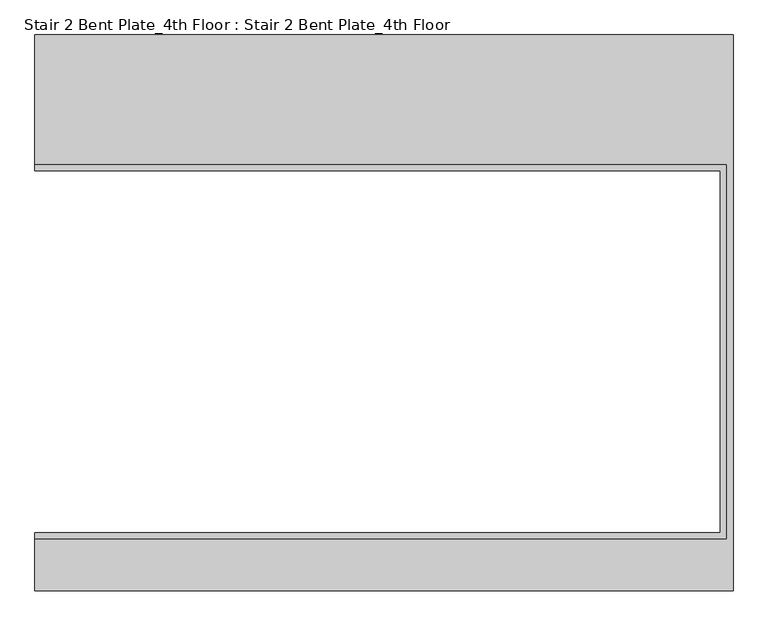
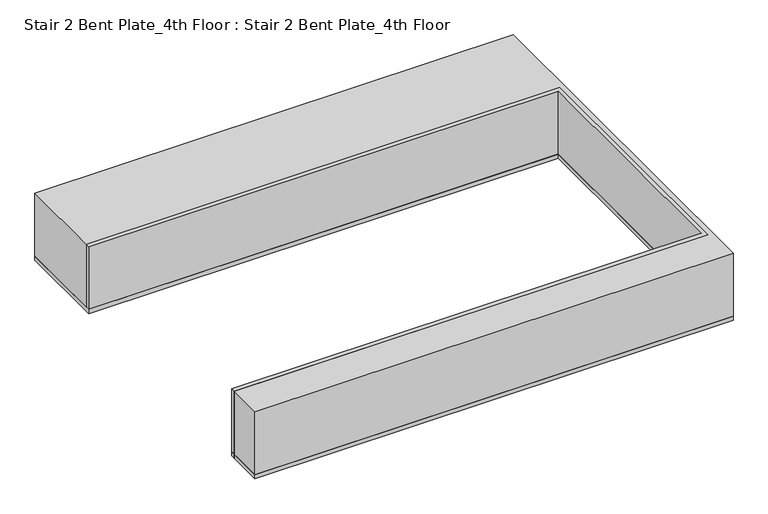
"""IFC4 building model written with IfcOpenShell, lengths in millimetres: proxy geometry, Stair 2 Bent Plate_4th Floor : Stair 2 Bent Plate_4th Floor."""

from ifc_helpers import new_model, si_unit, frame, origin, origin_with_axes, place, context, project, spatial, polyline, outline, extrude, source, transform, mapped, element, save


def stair_2_bent_plate_4th_floor_stair_2_bent_plate_4th_floor_69ec89e3(model_context):
    return source(origin(), model_context, "Body", "SweptSolid", [
        extrude(outline(polyline([(-247.65, -815.975), (-247.65, -714.375), (1111.25, -714.375), (1111.25, 22.225), (-247.65, 22.225), (-247.65, 276.225), (1123.95, 276.225), (1123.95, -815.975), (-247.65, -815.975)])), frame((0.0, 0.0, 12.7), z_axis=(0.0, 0.0, 1.0), x_axis=(1.0, 0.0, 0.0)), (0.0, 0.0, 1.0), 190.5),
        extrude(outline(polyline([(1123.95, -815.975), (-247.65, -815.975), (-247.65, -701.675), (1098.55, -701.675), (1098.55, 9.525), (-247.65, 9.525), (-247.65, 276.225), (1123.95, 276.225), (1123.95, -815.975)])), origin_with_axes(), (0.0, 0.0, 1.0), 12.7),
        extrude(outline(polyline([(-247.65, -701.675), (1098.55, -701.675), (1098.55, 9.525), (-247.65, 9.525), (-247.65, 22.225), (1111.25, 22.225), (1111.25, -714.375), (-247.65, -714.375), (-247.65, -701.675)])), origin_with_axes(), (0.0, 0.0, 1.0), 203.2),
    ])


if __name__ == "__main__":
    model = new_model("IFC4")
    model_context = context("Model", 3, world=origin())
    ifc_project = project(units=[si_unit("LENGTHUNIT", "METRE", prefix="MILLI")], contexts=[model_context])
    site = spatial("IfcSite", under=ifc_project)
    building = spatial("IfcBuilding", under=site)
    placement = place(None, origin())
    stair_2_bent_plate_4th_floor_stair_2_bent_plate_4th_floor_shape = stair_2_bent_plate_4th_floor_stair_2_bent_plate_4th_floor_69ec89e3(model_context)
    element("IfcBuildingElementProxy", 1, Name="Stair 2 Bent Plate_4th Floor : Stair 2 Bent Plate_4th Floor", ObjectType="Stair 2 Bent Plate_4th Floor : Stair 2 Bent Plate_4th Floor", at=placement, inside=building, context=model_context, shape_type="MappedRepresentation", body=[
        mapped(stair_2_bent_plate_4th_floor_stair_2_bent_plate_4th_floor_shape, transform((0.0, 0.0, 0.0), x_axis=(1.0, 0.0, 0.0), y_axis=(0.0, 1.0, 0.0), z_axis=(0.0, 0.0, 1.0))),
    ])
    save(model, "model.ifc")

# Revit data of these elements
# Element 1 (IfcBuildingElementProxy, "Stair 2 Bent Plate_4th Floor : Stair 2 Bent Plate_4th Floor")
#   Materials on its faces: "Concrete Infill"
# Materials
#   "Concrete Infill": class "Generic", colour RGB 0 255 0, transparency 0, Cost = 0
